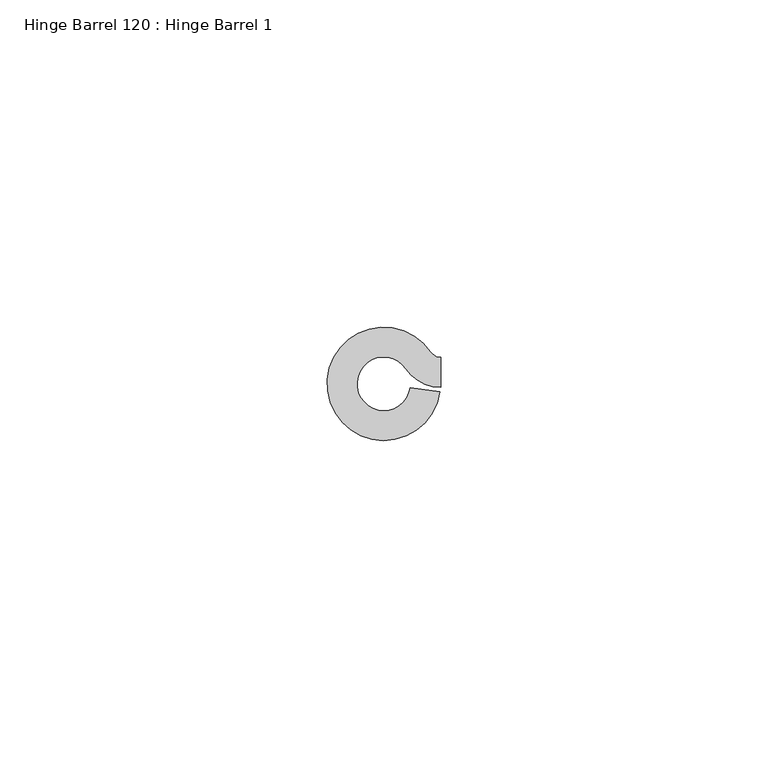
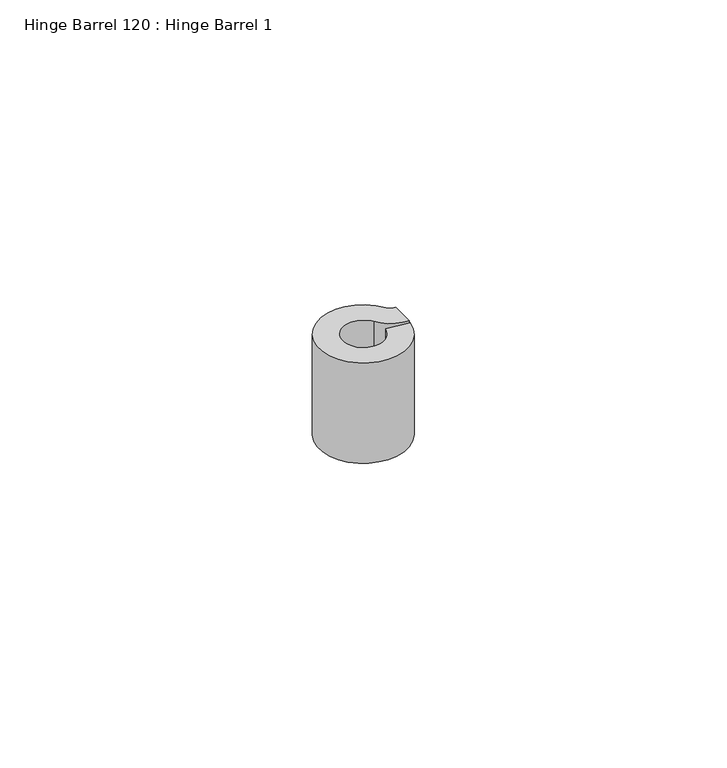
"""IFC4 building model written with IfcOpenShell, lengths in millimetres: proxy geometry, Hinge Barrel 120 : Hinge Barrel 1."""

import ifcopenshell
import ifcopenshell.guid

model = None  # the IFC model being written
_history = None  # IfcOwnerHistory: only IFC2X3 demands one
_inside = {}  # id of a spatial element -> (the spatial element, [elements in it])
_under = {}  # id of a project, library or spatial element -> (it, [spatial elements below it])
_declared = {}  # id of a project -> (the project, [libraries it declares])
_typed = {}  # id of a type object -> (the type object, [elements of that type])
_made_of = {}  # id of a material, layer set ... -> (it, [elements and type objects made of it])


def new_model(schema):
    """Start an empty IFC model of exactly this schema.

    Asked for "IFC4X3", IfcOpenShell would pick the latest addendum, in which some entities
    have other attributes; the version numbers below select the first issue.
    IFC2X3 requires an IfcOwnerHistory on every rooted entity: one is made here for all.
    """
    global model, _history
    if schema == "IFC4X3":
        model = ifcopenshell.file(schema_version=(4, 3, 0, 0))
    else:
        model = ifcopenshell.file(schema=schema)
    _inside.clear()
    _under.clear()
    _declared.clear()
    _typed.clear()
    _made_of.clear()
    _history = None
    if model.schema == "IFC2X3":
        org = make("IfcOrganization", Name="unknown")
        user = make(
            "IfcPersonAndOrganization",
            ThePerson=make("IfcPerson", FamilyName="unknown"),
            TheOrganization=org,
        )
        app = make(
            "IfcApplication",
            ApplicationDeveloper=org,
            Version="unknown",
            ApplicationFullName="unknown",
            ApplicationIdentifier="unknown",
        )
        _history = make(
            "IfcOwnerHistory",
            OwningUser=user,
            OwningApplication=app,
            ChangeAction="ADDED",
            CreationDate=0,
        )
    return model


def make(cls, **values):
    """One entity of the class cls with the attributes given. An attribute that is None is left unset."""
    return model.create_entity(
        cls, **{name: value for name, value in values.items() if value is not None}
    )


def rooted(cls, **values):
    """An entity with a GlobalId (a new one), such as an element, a storey or a relation."""
    return make(cls, GlobalId=ifcopenshell.guid.new(), OwnerHistory=_history, **values)


def si_unit(unit_type, name, prefix=None):
    """IfcSIUnit, for example si_unit("LENGTHUNIT", "METRE", prefix="MILLI")."""
    return make("IfcSIUnit", UnitType=unit_type, Prefix=prefix, Name=name)


def assignment(units):
    """IfcUnitAssignment: the units of a project."""
    return None if units is None else make("IfcUnitAssignment", Units=units)


def point(xyz):
    """IfcCartesianPoint."""
    return None if xyz is None else make("IfcCartesianPoint", Coordinates=xyz)


def direction(xyz):
    """IfcDirection."""
    return None if xyz is None else make("IfcDirection", DirectionRatios=xyz)


def frame(location, z_axis=None, x_axis=None):
    """IfcAxis2Placement3D, a coordinate frame: its origin and axes. An axis left out is left unset."""
    return make(
        "IfcAxis2Placement3D",
        Location=point(location),
        Axis=direction(z_axis),
        RefDirection=direction(x_axis),
    )


def frame_2d(location, x_axis=None):
    """IfcAxis2Placement2D, a coordinate frame in the plane: its origin and x axis."""
    return make(
        "IfcAxis2Placement2D", Location=point(location), RefDirection=direction(x_axis)
    )


def origin():
    """The frame at (0, 0, 0) with its axes left unset."""
    return frame((0.0, 0.0, 0.0))


def place(relative_to, where):
    """IfcLocalPlacement: puts the frame where relative to a parent placement (None: the world)."""
    return make(
        "IfcLocalPlacement", PlacementRelTo=relative_to, RelativePlacement=where
    )


def context(
    kind, dimensions, precision=None, world=None, true_north=None, identifier=None
):
    """IfcGeometricRepresentationContext, for example the 3D "Model" context."""
    return make(
        "IfcGeometricRepresentationContext",
        ContextIdentifier=identifier,
        ContextType=kind,
        CoordinateSpaceDimension=dimensions,
        Precision=precision,
        WorldCoordinateSystem=world,
        TrueNorth=true_north,
    )


def project(units=None, contexts=None):
    """IfcProject with its units and contexts."""
    return rooted(
        "IfcProject",
        Name="project",
        RepresentationContexts=contexts,
        UnitsInContext=assignment(units),
    )


def spatial(cls, under=None, at=None, **own):
    """A site, building, storey or space (cls), placed at a placement, below another one or the project."""
    s = rooted(cls, ObjectPlacement=at, **own)
    if under is not None:
        _under.setdefault(under.id(), (under, []))[1].append(s)
    return s


def polyline(points):
    """IfcPolyline through the points."""
    return make("IfcPolyline", Points=[point(p) for p in points])


def circle_curve(where, radius):
    """IfcCircle in the frame where."""
    return make("IfcCircle", Position=where, Radius=radius)


def trimmed(basis, trim1, trim2, sense, master):
    """IfcTrimmedCurve: the piece of a basis curve between two trims."""
    return make(
        "IfcTrimmedCurve",
        BasisCurve=basis,
        Trim1=trim1,
        Trim2=trim2,
        SenseAgreement=sense,
        MasterRepresentation=master,
    )


def segment(curve, same_sense, transition):
    """IfcCompositeCurveSegment."""
    return make(
        "IfcCompositeCurveSegment",
        Transition=transition,
        SameSense=same_sense,
        ParentCurve=curve,
    )


def composite_curve(segments, self_intersect=None):
    """IfcCompositeCurve: segments joined end to end."""
    return make("IfcCompositeCurve", Segments=segments, SelfIntersect=self_intersect)


def outline(outer, holes=None, kind="AREA"):
    """IfcArbitraryClosedProfileDef: a profile drawn as a closed curve; with holes, ...WithVoids."""
    if holes is None:
        return make("IfcArbitraryClosedProfileDef", ProfileType=kind, OuterCurve=outer)
    return make(
        "IfcArbitraryProfileDefWithVoids",
        ProfileType=kind,
        OuterCurve=outer,
        InnerCurves=holes,
    )


def extrude(swept, where, along, depth):
    """IfcExtrudedAreaSolid: the profile swept, set in the frame where, extruded along a direction by depth."""
    return make(
        "IfcExtrudedAreaSolid",
        SweptArea=swept,
        Position=where,
        ExtrudedDirection=direction(along),
        Depth=depth,
    )


def shape(context_of_items, identifier, shape_type, items):
    """IfcShapeRepresentation: the items that make up one representation, for example the "Body"."""
    return make(
        "IfcShapeRepresentation",
        ContextOfItems=context_of_items,
        RepresentationIdentifier=identifier,
        RepresentationType=shape_type,
        Items=items,
    )


def source(mapping_origin, context_of_items, identifier, shape_type, items):
    """IfcRepresentationMap: a shape defined once, which mapped items show again and again."""
    return make(
        "IfcRepresentationMap",
        MappingOrigin=mapping_origin,
        MappedRepresentation=shape(context_of_items, identifier, shape_type, items),
    )


def transform(
    local_origin,
    x_axis=None,
    y_axis=None,
    z_axis=None,
    scale=None,
    scale2=None,
    scale3=None,
    uniform=True,
):
    """IfcCartesianTransformationOperator3D, or its non-uniform kind. x_axis, y_axis, z_axis: its Axis1, 2, 3."""
    if uniform:
        return make(
            "IfcCartesianTransformationOperator3D",
            Axis1=direction(x_axis),
            Axis2=direction(y_axis),
            LocalOrigin=point(local_origin),
            Scale=scale,
            Axis3=direction(z_axis),
        )
    return make(
        "IfcCartesianTransformationOperator3DnonUniform",
        Axis1=direction(x_axis),
        Axis2=direction(y_axis),
        LocalOrigin=point(local_origin),
        Scale=scale,
        Axis3=direction(z_axis),
        Scale2=scale2,
        Scale3=scale3,
    )


def mapped(mapping_source, mapping_target):
    """IfcMappedItem: shows the shape of a source again, moved by a transform."""
    return make(
        "IfcMappedItem", MappingSource=mapping_source, MappingTarget=mapping_target
    )


def made_of(thing, what):
    """Note that an element or type object is made of a material, layer set ...; save() writes the relation."""
    if what is not None:
        _made_of.setdefault(what.id(), (what, []))[1].append(thing)
    return thing


def element(
    cls,
    number,
    at=None,
    inside=None,
    cuts=None,
    type_object=None,
    material=None,
    context=None,
    identifier="Body",
    shape_type=None,
    held_by="IfcProductDefinitionShape",
    body=None,
    shapes=None,
    **own,
):
    """One element of the class cls, such as IfcWall. Its Tag is "e" and its number.

    at: its placement. inside: the storey or other place that contains it. cuts: it is an
    opening in that element (IfcRelVoidsElement). A single representation is given by context,
    identifier, shape_type and body (its items); several are given by shapes. held_by: the class
    of the entity that holds the representations. save() writes the other relations.
    """
    e = rooted(cls, Tag="e%d" % number, ObjectPlacement=at, **own)
    if body is not None:
        shapes = [shape(context, identifier, shape_type, body)]
    if shapes is not None:
        e.Representation = make(held_by, Representations=shapes)
    if inside is not None:
        _inside.setdefault(inside.id(), (inside, []))[1].append(e)
    if cuts is not None:
        rooted(
            "IfcRelVoidsElement", RelatingBuildingElement=cuts, RelatedOpeningElement=e
        )
    if type_object is not None:
        _typed.setdefault(type_object.id(), (type_object, []))[1].append(e)
    return made_of(e, material)


def aggregate(whole, parts):
    """IfcRelAggregates: a whole, such as a stair, and the parts it consists of."""
    return rooted("IfcRelAggregates", RelatingObject=whole, RelatedObjects=parts)


def save(model, path):
    """Write the relations noted so far, then the file.

    IfcRelAggregates (storeys below a building ...), IfcRelContainedInSpatialStructure (elements
    in a storey), IfcRelDefinesByType, IfcRelAssociatesMaterial and IfcRelDeclares: one each for
    every whole, place, type object, material and project.
    """
    for whole, parts in _under.values():
        aggregate(whole, parts)
    for where, things in _inside.values():
        rooted(
            "IfcRelContainedInSpatialStructure",
            RelatedElements=things,
            RelatingStructure=where,
        )
    for kind, things in _typed.values():
        rooted("IfcRelDefinesByType", RelatedObjects=things, RelatingType=kind)
    for what, things in _made_of.values():
        rooted("IfcRelAssociatesMaterial", RelatedObjects=things, RelatingMaterial=what)
    for by, libraries in _declared.values():
        rooted("IfcRelDeclares", RelatingContext=by, RelatedDefinitions=libraries)
    model.write(path)


def hinge_barrel_120_hinge_barrel_1_1e94fffa(model_context):
    return source(origin(), model_context, "Body", "SweptSolid", [
        extrude(outline(composite_curve([segment(trimmed(circle_curve(frame_2d((587319.1320739, -534100.7049841)), 4.0894), [point((587322.5194669, -534098.4139665))], [point((587323.1821338, -534101.2708529))], True, "CARTESIAN"), True, "CONTINUOUS"), segment(polyline([(587323.1821338, -534101.2708529), (587327.7022899, -534101.9024028)]), True, "CONTINUOUS"), segment(trimmed(circle_curve(frame_2d((587319.1320739, -534100.7049841)), 8.6534625), [point((587327.7022899, -534101.9024028))], [point((587326.3000393, -534095.8570273))], False, "CARTESIAN"), True, "CONTINUOUS"), segment(trimmed(circle_curve(frame_2d((587327.8245257, -534094.8259615)), 1.8404226), [point((587326.3000393, -534095.8570273))], [point((587327.8245257, -534096.6663841))], True, "CARTESIAN"), True, "CONTINUOUS"), segment(polyline([(587327.8245257, -534096.6663841), (587327.8245257, -534101.2304466)]), True, "CONTINUOUS"), segment(trimmed(circle_curve(frame_2d((587327.8245257, -534094.8259615)), 6.4044851), [point((587327.8245257, -534101.2304466))], [point((587322.5194669, -534098.4139665))], False, "CARTESIAN"), True, "CONTINUOUS")], self_intersect=False)), frame((0.0, 0.0, 2063.75), z_axis=(0.0, 0.0, 1.0), x_axis=(1.0, 0.0, 0.0)), (0.0, 0.0, 1.0), 20.8359375),
    ])


if __name__ == "__main__":
    model = new_model("IFC4")
    model_context = context("Model", 3, world=origin())
    ifc_project = project(units=[si_unit("LENGTHUNIT", "METRE", prefix="MILLI")], contexts=[model_context])
    site = spatial("IfcSite", under=ifc_project)
    building = spatial("IfcBuilding", under=site)
    placement = place(None, origin())
    hinge_barrel_120_hinge_barrel_1_shape = hinge_barrel_120_hinge_barrel_1_1e94fffa(model_context)
    element("IfcBuildingElementProxy", 1, Name="Hinge Barrel 120 : Hinge Barrel 1", ObjectType="Hinge Barrel 120 : Hinge Barrel 1", at=placement, inside=building, context=model_context, shape_type="MappedRepresentation", body=[
        mapped(hinge_barrel_120_hinge_barrel_1_shape, transform((0.0, 0.0, 0.0), x_axis=(1.0, 0.0, 0.0), y_axis=(0.0, 1.0, 0.0), z_axis=(0.0, 0.0, 1.0))),
    ])
    save(model, "model.ifc")

# Revit data of these elements
# Element 1 (IfcBuildingElementProxy, "Hinge Barrel 120 : Hinge Barrel 1")
#   Materials on its faces: "6\"X6\" WELD-ON STL BUTT HINGE"
# Materials
#   "6\"X6\" WELD-ON STL BUTT HINGE": class "Metal", colour RGB 189 187 185, transparency 0, Description = "Carbon steel", Cost = 0
